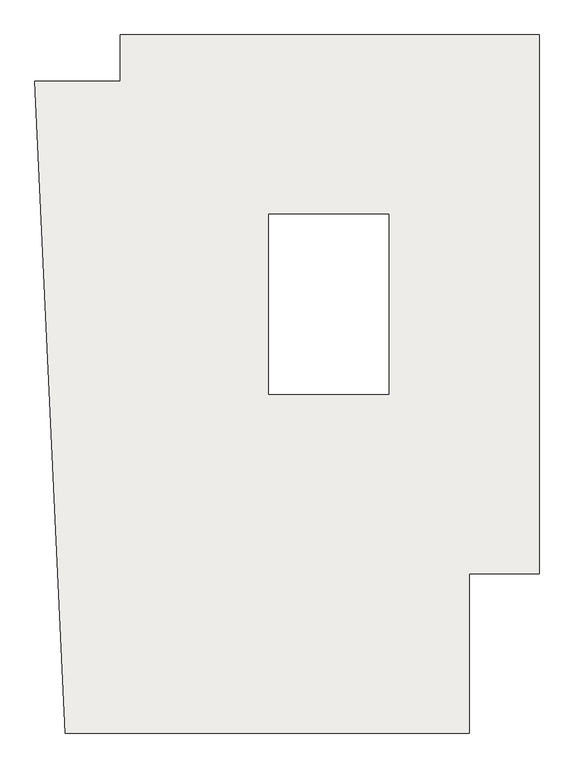
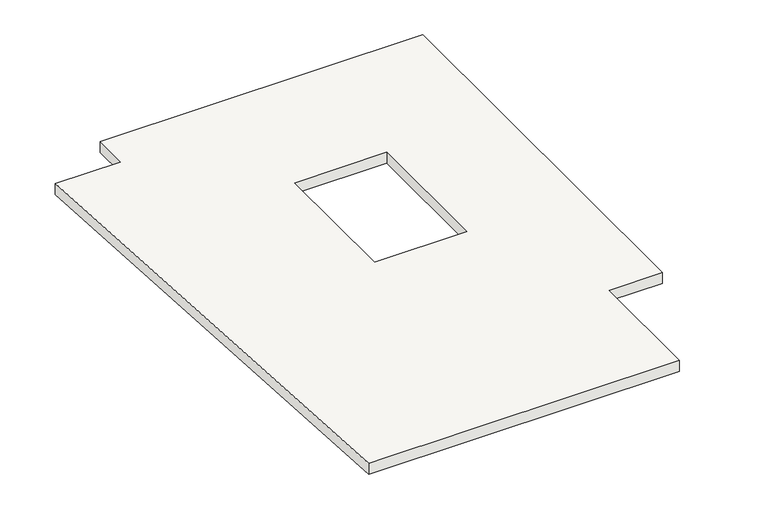
"""IFC4 building model written with IfcOpenShell, lengths in millimetres: slab geometry, Holzdecke : Holzdecke."""

from ifc_helpers import new_model, si_unit, frame, origin, place, context, project, spatial, polyline, outline, extrude, source, transform, mapped, element, save


def slab_df54632a(model_context):
    return source(origin(), model_context, "Body", "SweptSolid", [
        extrude(outline(polyline([(156973.3526125, 23156.8751908), (155952.5612199, 44944.1136987), (158797.7593015, 44944.1136987), (158797.7593015, 46484.7962965), (172797.7593015, 46484.7962965), (172797.7593015, 28481.9343946), (170467.7593015, 28481.9343946), (170467.7593015, 23156.8751908), (156973.3526125, 23156.8751908)]), holes=[polyline([(167772.7593015, 40484.7962965), (163772.7593015, 40484.7962965), (163772.7593015, 34484.7962965), (167772.7593015, 34484.7962965), (167772.7593015, 40484.7962965)])]), frame((0.0, 0.0, -500.0), z_axis=(0.0, 0.0, 1.0), x_axis=(1.0, 0.0, 0.0)), (0.0, 0.0, 1.0), 500.0),
    ])


if __name__ == "__main__":
    model = new_model("IFC4")
    model_context = context("Model", 3, world=origin())
    ifc_project = project(units=[si_unit("LENGTHUNIT", "METRE", prefix="MILLI")], contexts=[model_context])
    site = spatial("IfcSite", under=ifc_project)
    building = spatial("IfcBuilding", under=site)
    placement = place(None, origin())
    slab_shape = slab_df54632a(model_context)
    element("IfcSlab", 1, ObjectType="Holzdecke : Holzdecke", at=placement, inside=building, context=model_context, shape_type="MappedRepresentation", body=[
        mapped(slab_shape, transform((0.0, 0.0, 0.0), x_axis=(1.0, 0.0, 0.0), y_axis=(0.0, 1.0, 0.0), z_axis=(0.0, 0.0, 1.0))),
    ])
    save(model, "model.ifc")

# Revit data of these elements
# Type "Holzdecke : Holzdecke"
#   Abrechnungsart = "m²"
#   Allright_Bauteil_ID = "0110De 0783954323"
#   Bezeichnung = "Holzdecke"
#   Codetext = "D-HOLZBALKEN1\\"
#   Gewerk = "Zimmer- und Holzbauarbeiten"
#   Material = "Holz"
#   Objektname = "Brettstapeldecke"
#   NameOverride = "Holzdecke"
#   Reference = "Holzdecke"
#   Status = "NEW"
#   PitchAngle = 0.00°
#   ThermalTransmittance = 0.0000 BTU/(h·ft²·°F)
#   2D Interaktion = yes
#   Combustible = no
#   Compartmentation = no
#   IsExternal = no
#   LoadBearing = yes
# Element 1 (IfcSlab, "Holzdecke : Holzdecke")
#   Materials on its faces: "Default Floor"
# Materials
#   "Default Floor": class "Miscellaneous", colour RGB 128 128 128, transparency 0, Cost = 0
